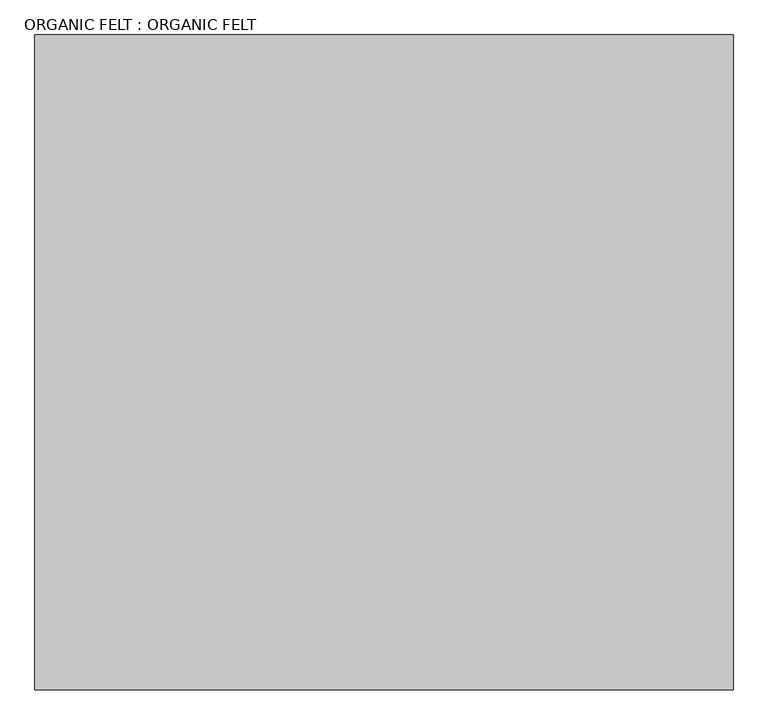
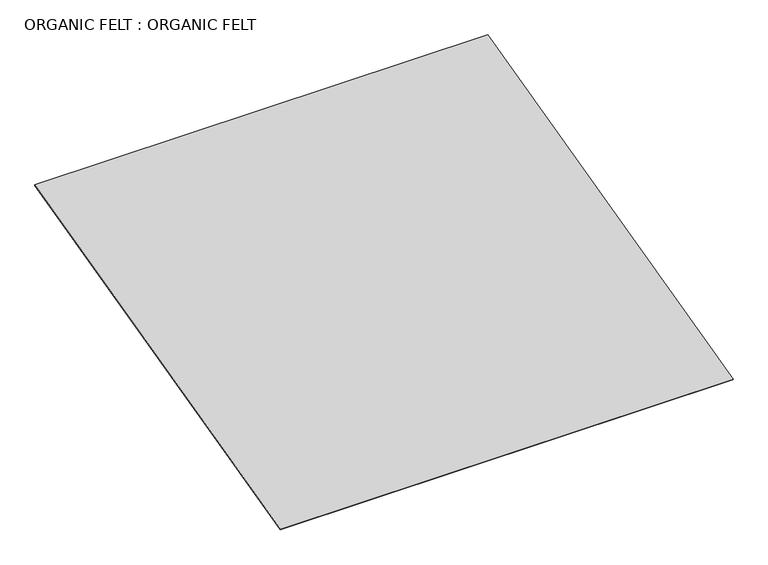
"""IFC4 building model written with IfcOpenShell, lengths in millimetres: proxy geometry, ORGANIC FELT : ORGANIC FELT."""

import ifcopenshell
import ifcopenshell.guid

model = None  # the IFC model being written
_history = None  # IfcOwnerHistory: only IFC2X3 demands one
_inside = {}  # id of a spatial element -> (the spatial element, [elements in it])
_under = {}  # id of a project, library or spatial element -> (it, [spatial elements below it])
_declared = {}  # id of a project -> (the project, [libraries it declares])
_typed = {}  # id of a type object -> (the type object, [elements of that type])
_made_of = {}  # id of a material, layer set ... -> (it, [elements and type objects made of it])


def new_model(schema):
    """Start an empty IFC model of exactly this schema.

    Asked for "IFC4X3", IfcOpenShell would pick the latest addendum, in which some entities
    have other attributes; the version numbers below select the first issue.
    IFC2X3 requires an IfcOwnerHistory on every rooted entity: one is made here for all.
    """
    global model, _history
    if schema == "IFC4X3":
        model = ifcopenshell.file(schema_version=(4, 3, 0, 0))
    else:
        model = ifcopenshell.file(schema=schema)
    _inside.clear()
    _under.clear()
    _declared.clear()
    _typed.clear()
    _made_of.clear()
    _history = None
    if model.schema == "IFC2X3":
        org = make("IfcOrganization", Name="unknown")
        user = make(
            "IfcPersonAndOrganization",
            ThePerson=make("IfcPerson", FamilyName="unknown"),
            TheOrganization=org,
        )
        app = make(
            "IfcApplication",
            ApplicationDeveloper=org,
            Version="unknown",
            ApplicationFullName="unknown",
            ApplicationIdentifier="unknown",
        )
        _history = make(
            "IfcOwnerHistory",
            OwningUser=user,
            OwningApplication=app,
            ChangeAction="ADDED",
            CreationDate=0,
        )
    return model


def make(cls, **values):
    """One entity of the class cls with the attributes given. An attribute that is None is left unset."""
    return model.create_entity(
        cls, **{name: value for name, value in values.items() if value is not None}
    )


def rooted(cls, **values):
    """An entity with a GlobalId (a new one), such as an element, a storey or a relation."""
    return make(cls, GlobalId=ifcopenshell.guid.new(), OwnerHistory=_history, **values)


def si_unit(unit_type, name, prefix=None):
    """IfcSIUnit, for example si_unit("LENGTHUNIT", "METRE", prefix="MILLI")."""
    return make("IfcSIUnit", UnitType=unit_type, Prefix=prefix, Name=name)


def assignment(units):
    """IfcUnitAssignment: the units of a project."""
    return None if units is None else make("IfcUnitAssignment", Units=units)


def point(xyz):
    """IfcCartesianPoint."""
    return None if xyz is None else make("IfcCartesianPoint", Coordinates=xyz)


def direction(xyz):
    """IfcDirection."""
    return None if xyz is None else make("IfcDirection", DirectionRatios=xyz)


def frame(location, z_axis=None, x_axis=None):
    """IfcAxis2Placement3D, a coordinate frame: its origin and axes. An axis left out is left unset."""
    return make(
        "IfcAxis2Placement3D",
        Location=point(location),
        Axis=direction(z_axis),
        RefDirection=direction(x_axis),
    )


def origin():
    """The frame at (0, 0, 0) with its axes left unset."""
    return frame((0.0, 0.0, 0.0))


def place(relative_to, where):
    """IfcLocalPlacement: puts the frame where relative to a parent placement (None: the world)."""
    return make(
        "IfcLocalPlacement", PlacementRelTo=relative_to, RelativePlacement=where
    )


def context(
    kind, dimensions, precision=None, world=None, true_north=None, identifier=None
):
    """IfcGeometricRepresentationContext, for example the 3D "Model" context."""
    return make(
        "IfcGeometricRepresentationContext",
        ContextIdentifier=identifier,
        ContextType=kind,
        CoordinateSpaceDimension=dimensions,
        Precision=precision,
        WorldCoordinateSystem=world,
        TrueNorth=true_north,
    )


def project(units=None, contexts=None):
    """IfcProject with its units and contexts."""
    return rooted(
        "IfcProject",
        Name="project",
        RepresentationContexts=contexts,
        UnitsInContext=assignment(units),
    )


def spatial(cls, under=None, at=None, **own):
    """A site, building, storey or space (cls), placed at a placement, below another one or the project."""
    s = rooted(cls, ObjectPlacement=at, **own)
    if under is not None:
        _under.setdefault(under.id(), (under, []))[1].append(s)
    return s


def polyline(points):
    """IfcPolyline through the points."""
    return make("IfcPolyline", Points=[point(p) for p in points])


def outline(outer, holes=None, kind="AREA"):
    """IfcArbitraryClosedProfileDef: a profile drawn as a closed curve; with holes, ...WithVoids."""
    if holes is None:
        return make("IfcArbitraryClosedProfileDef", ProfileType=kind, OuterCurve=outer)
    return make(
        "IfcArbitraryProfileDefWithVoids",
        ProfileType=kind,
        OuterCurve=outer,
        InnerCurves=holes,
    )


def extrude(swept, where, along, depth):
    """IfcExtrudedAreaSolid: the profile swept, set in the frame where, extruded along a direction by depth."""
    return make(
        "IfcExtrudedAreaSolid",
        SweptArea=swept,
        Position=where,
        ExtrudedDirection=direction(along),
        Depth=depth,
    )


def shape(context_of_items, identifier, shape_type, items):
    """IfcShapeRepresentation: the items that make up one representation, for example the "Body"."""
    return make(
        "IfcShapeRepresentation",
        ContextOfItems=context_of_items,
        RepresentationIdentifier=identifier,
        RepresentationType=shape_type,
        Items=items,
    )


def source(mapping_origin, context_of_items, identifier, shape_type, items):
    """IfcRepresentationMap: a shape defined once, which mapped items show again and again."""
    return make(
        "IfcRepresentationMap",
        MappingOrigin=mapping_origin,
        MappedRepresentation=shape(context_of_items, identifier, shape_type, items),
    )


def transform(
    local_origin,
    x_axis=None,
    y_axis=None,
    z_axis=None,
    scale=None,
    scale2=None,
    scale3=None,
    uniform=True,
):
    """IfcCartesianTransformationOperator3D, or its non-uniform kind. x_axis, y_axis, z_axis: its Axis1, 2, 3."""
    if uniform:
        return make(
            "IfcCartesianTransformationOperator3D",
            Axis1=direction(x_axis),
            Axis2=direction(y_axis),
            LocalOrigin=point(local_origin),
            Scale=scale,
            Axis3=direction(z_axis),
        )
    return make(
        "IfcCartesianTransformationOperator3DnonUniform",
        Axis1=direction(x_axis),
        Axis2=direction(y_axis),
        LocalOrigin=point(local_origin),
        Scale=scale,
        Axis3=direction(z_axis),
        Scale2=scale2,
        Scale3=scale3,
    )


def mapped(mapping_source, mapping_target):
    """IfcMappedItem: shows the shape of a source again, moved by a transform."""
    return make(
        "IfcMappedItem", MappingSource=mapping_source, MappingTarget=mapping_target
    )


def made_of(thing, what):
    """Note that an element or type object is made of a material, layer set ...; save() writes the relation."""
    if what is not None:
        _made_of.setdefault(what.id(), (what, []))[1].append(thing)
    return thing


def element(
    cls,
    number,
    at=None,
    inside=None,
    cuts=None,
    type_object=None,
    material=None,
    context=None,
    identifier="Body",
    shape_type=None,
    held_by="IfcProductDefinitionShape",
    body=None,
    shapes=None,
    **own,
):
    """One element of the class cls, such as IfcWall. Its Tag is "e" and its number.

    at: its placement. inside: the storey or other place that contains it. cuts: it is an
    opening in that element (IfcRelVoidsElement). A single representation is given by context,
    identifier, shape_type and body (its items); several are given by shapes. held_by: the class
    of the entity that holds the representations. save() writes the other relations.
    """
    e = rooted(cls, Tag="e%d" % number, ObjectPlacement=at, **own)
    if body is not None:
        shapes = [shape(context, identifier, shape_type, body)]
    if shapes is not None:
        e.Representation = make(held_by, Representations=shapes)
    if inside is not None:
        _inside.setdefault(inside.id(), (inside, []))[1].append(e)
    if cuts is not None:
        rooted(
            "IfcRelVoidsElement", RelatingBuildingElement=cuts, RelatedOpeningElement=e
        )
    if type_object is not None:
        _typed.setdefault(type_object.id(), (type_object, []))[1].append(e)
    return made_of(e, material)


def aggregate(whole, parts):
    """IfcRelAggregates: a whole, such as a stair, and the parts it consists of."""
    return rooted("IfcRelAggregates", RelatingObject=whole, RelatedObjects=parts)


def save(model, path):
    """Write the relations noted so far, then the file.

    IfcRelAggregates (storeys below a building ...), IfcRelContainedInSpatialStructure (elements
    in a storey), IfcRelDefinesByType, IfcRelAssociatesMaterial and IfcRelDeclares: one each for
    every whole, place, type object, material and project.
    """
    for whole, parts in _under.values():
        aggregate(whole, parts)
    for where, things in _inside.values():
        rooted(
            "IfcRelContainedInSpatialStructure",
            RelatedElements=things,
            RelatingStructure=where,
        )
    for kind, things in _typed.values():
        rooted("IfcRelDefinesByType", RelatedObjects=things, RelatingType=kind)
    for what, things in _made_of.values():
        rooted("IfcRelAssociatesMaterial", RelatedObjects=things, RelatingMaterial=what)
    for by, libraries in _declared.values():
        rooted("IfcRelDeclares", RelatingContext=by, RelatedDefinitions=libraries)
    model.write(path)


def organic_felt_organic_felt_21a7ef86(model_context):
    return source(origin(), model_context, "Body", "SweptSolid", [
        extrude(outline(polyline([(-5223.7687621, 42827.1220986), (-3345.9908907, 43296.5665664), (-3345.9908907, 43293.2938513), (-5222.9987115, 42824.0418961), (-5223.7687621, 42827.1220986)])), frame((12382.7678845, 0.0, 0.0), z_axis=(1.0, 0.0, 0.0), x_axis=(0.0, 1.0, 0.0)), (0.0, 0.0, 1.0), 2000.25),
    ])


if __name__ == "__main__":
    model = new_model("IFC4")
    model_context = context("Model", 3, world=origin())
    ifc_project = project(units=[si_unit("LENGTHUNIT", "METRE", prefix="MILLI")], contexts=[model_context])
    site = spatial("IfcSite", under=ifc_project)
    building = spatial("IfcBuilding", under=site)
    placement = place(None, origin())
    organic_felt_organic_felt_shape = organic_felt_organic_felt_21a7ef86(model_context)
    element("IfcBuildingElementProxy", 1, Name="ORGANIC FELT : ORGANIC FELT", ObjectType="ORGANIC FELT : ORGANIC FELT", at=placement, inside=building, context=model_context, shape_type="MappedRepresentation", body=[
        mapped(organic_felt_organic_felt_shape, transform((0.0, 0.0, 0.0), x_axis=(1.0, 0.0, 0.0), y_axis=(0.0, 1.0, 0.0), z_axis=(0.0, 0.0, 1.0))),
    ])
    save(model, "model.ifc")

# Revit data of these elements
# Type "ORGANIC FELT : ORGANIC FELT"
#   NameOverride = "ORGANIC FELT"
# Element 1 (IfcBuildingElementProxy, "ORGANIC FELT : ORGANIC FELT")
#   Materials on its faces: "ASPHALT SATURATED ORGANIC FELT @ ROOF"
# Materials
#   "ASPHALT SATURATED ORGANIC FELT @ ROOF": class "Unassigned", colour RGB 85 170 127, transparency 0
